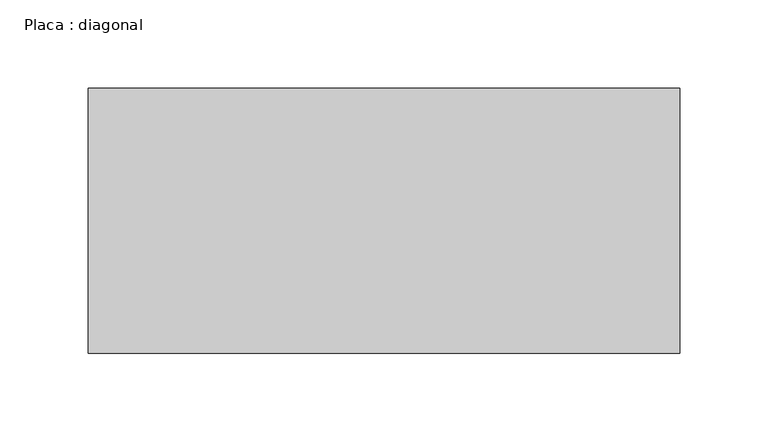
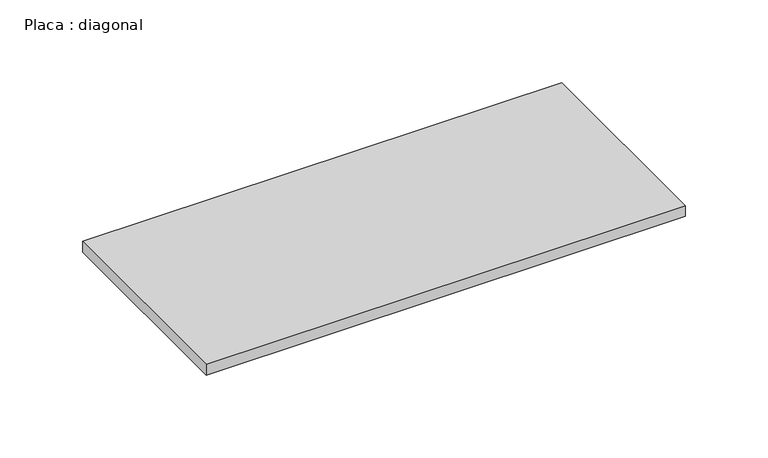
"""IFC4 building model written with IfcOpenShell, lengths in millimetres: beam geometry, Placa : diagonal."""

from ifc_helpers import new_model, si_unit, frame, origin, place, context, project, spatial, polyline, outline, extrude, source, transform, mapped, element, save


def placa_diagonal_7c75d2cc(model_context):
    return source(origin(), model_context, "Body", "SweptSolid", [
        extrude(outline(polyline([(167.0043072, 75.0), (167.0043072, -75.0), (-167.7829143, -75.0), (-167.7829143, 75.0), (167.0043072, 75.0)])), frame((0.0, 0.0, -4.0), z_axis=(0.0, 0.0, 1.0), x_axis=(1.0, 0.0, 0.0)), (0.0, 0.0, 1.0), 8.0),
    ])


if __name__ == "__main__":
    model = new_model("IFC4")
    model_context = context("Model", 3, world=origin())
    ifc_project = project(units=[si_unit("LENGTHUNIT", "METRE", prefix="MILLI")], contexts=[model_context])
    site = spatial("IfcSite", under=ifc_project)
    building = spatial("IfcBuilding", under=site)
    placement = place(None, origin())
    placa_diagonal_shape = placa_diagonal_7c75d2cc(model_context)
    element("IfcBeam", 1, ObjectType="Placa : diagonal", at=placement, inside=building, context=model_context, shape_type="MappedRepresentation", body=[
        mapped(placa_diagonal_shape, transform((0.0, 0.0, 0.0), x_axis=(1.0, 0.0, 0.0), y_axis=(0.0, 1.0, 0.0), z_axis=(0.0, 0.0, 1.0))),
    ])
    save(model, "model.ifc")

# Revit data of these elements
# Type "Placa : diagonal"
#   W = 0
#   Length [instance default] = 1.50 m
#   b = 0.15 m
#   d = 0.008 m
#   A = 0 m²
#   Structural Material [instance default] = Aço, 45-345
# Element 1 (IfcBeam, "Placa : diagonal")
#   Materials on its faces: "Aço, 45-345"
# Materials
#   "Aço, 45-345": class "Metal", colour RGB 247 247 247, transparency 0, Description = "Aço 345 MPa", Cost = 0
